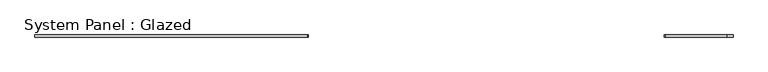
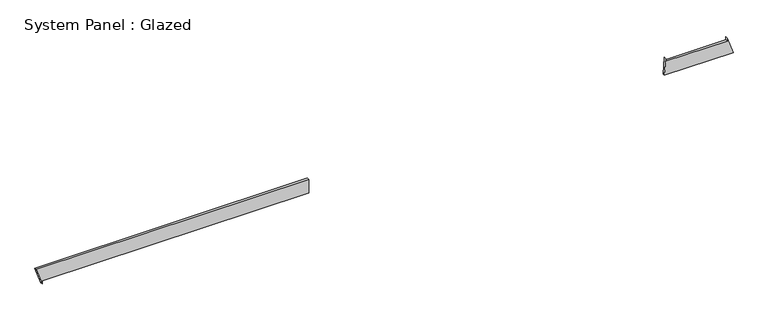
"""IFC4 building model written with IfcOpenShell, lengths in millimetres: plate geometry, System Panel : Glazed."""

from ifc_helpers import new_model, si_unit, frame, origin, place, context, project, spatial, polyline, outline, extrude, source, transform, mapped, element, save


def system_panel_glazed_dba537f6(model_context):
    return source(origin(), model_context, "Body", "SweptSolid", [
        extrude(outline(polyline([(35.3553391, 3233.2334966), (35.3553391, 4027.7930193), (235.7005018, 3958.9828813), (200.3451627, 3958.98343), (200.3341084, 3246.7911885), (235.6894474, 3246.7906397), (35.3553391, 3233.2334966)])), frame((0.0, -49.5, 0.0), z_axis=(0.0, 1.0, 0.0), x_axis=(0.0, 0.0, 1.0)), (0.0, 0.0, 1.0), 25.0),
        extrude(outline(polyline([(0.0, -3958.6827411), (35.3553391, -3958.6827411), (35.3553391, -875.2968038), (200.2700807, -878.2816654), (200.2211953, -4027.7930193), (0.0, -3958.6827411)])), frame((0.0, -49.5, 0.0), z_axis=(0.0, 1.0, 0.0), x_axis=(0.0, 0.0, 1.0)), (0.0, 0.0, 1.0), 25.0),
    ])


if __name__ == "__main__":
    model = new_model("IFC4")
    model_context = context("Model", 3, world=origin())
    ifc_project = project(units=[si_unit("LENGTHUNIT", "METRE", prefix="MILLI")], contexts=[model_context])
    site = spatial("IfcSite", under=ifc_project)
    building = spatial("IfcBuilding", under=site)
    placement = place(None, origin())
    system_panel_glazed_shape = system_panel_glazed_dba537f6(model_context)
    element("IfcPlate", 1, ObjectType="System Panel : Glazed", at=placement, inside=building, context=model_context, shape_type="MappedRepresentation", body=[
        mapped(system_panel_glazed_shape, transform((0.0, 0.0, 0.0), x_axis=(1.0, 0.0, 0.0), y_axis=(0.0, 1.0, 0.0), z_axis=(0.0, 0.0, 1.0))),
    ])
    save(model, "model.ifc")

# Revit data of these elements
# Element 1 (IfcPlate, "System Panel : Glazed")
#   Materials on its faces: "Glass"
# Materials
#   "Glass": class "Glass", colour RGB 218 227 224, transparency 0.85, Description = "Soda Lime Glass", Cost = 0
